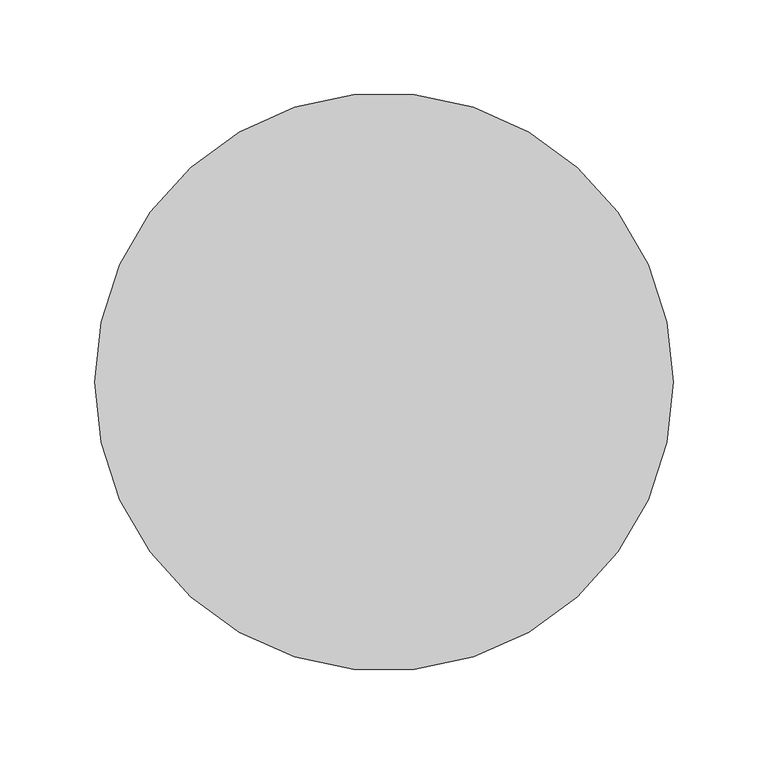
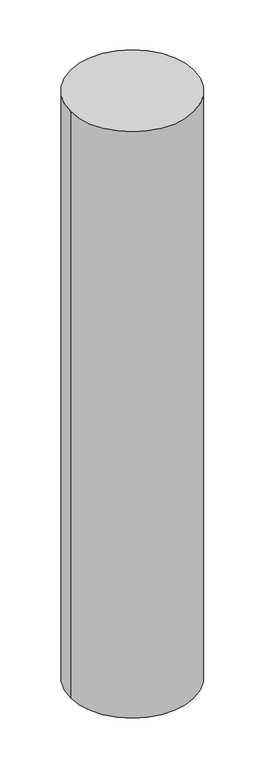
"""IFC4 building model written with IfcOpenShell, lengths in millimetres: proxy geometry."""

import ifcopenshell
import ifcopenshell.guid

model = None  # the IFC model being written
_history = None  # IfcOwnerHistory: only IFC2X3 demands one
_inside = {}  # id of a spatial element -> (the spatial element, [elements in it])
_under = {}  # id of a project, library or spatial element -> (it, [spatial elements below it])
_declared = {}  # id of a project -> (the project, [libraries it declares])
_typed = {}  # id of a type object -> (the type object, [elements of that type])
_made_of = {}  # id of a material, layer set ... -> (it, [elements and type objects made of it])


def new_model(schema):
    """Start an empty IFC model of exactly this schema.

    Asked for "IFC4X3", IfcOpenShell would pick the latest addendum, in which some entities
    have other attributes; the version numbers below select the first issue.
    IFC2X3 requires an IfcOwnerHistory on every rooted entity: one is made here for all.
    """
    global model, _history
    if schema == "IFC4X3":
        model = ifcopenshell.file(schema_version=(4, 3, 0, 0))
    else:
        model = ifcopenshell.file(schema=schema)
    _inside.clear()
    _under.clear()
    _declared.clear()
    _typed.clear()
    _made_of.clear()
    _history = None
    if model.schema == "IFC2X3":
        org = make("IfcOrganization", Name="unknown")
        user = make(
            "IfcPersonAndOrganization",
            ThePerson=make("IfcPerson", FamilyName="unknown"),
            TheOrganization=org,
        )
        app = make(
            "IfcApplication",
            ApplicationDeveloper=org,
            Version="unknown",
            ApplicationFullName="unknown",
            ApplicationIdentifier="unknown",
        )
        _history = make(
            "IfcOwnerHistory",
            OwningUser=user,
            OwningApplication=app,
            ChangeAction="ADDED",
            CreationDate=0,
        )
    return model


def make(cls, **values):
    """One entity of the class cls with the attributes given. An attribute that is None is left unset."""
    return model.create_entity(
        cls, **{name: value for name, value in values.items() if value is not None}
    )


def rooted(cls, **values):
    """An entity with a GlobalId (a new one), such as an element, a storey or a relation."""
    return make(cls, GlobalId=ifcopenshell.guid.new(), OwnerHistory=_history, **values)


def si_unit(unit_type, name, prefix=None):
    """IfcSIUnit, for example si_unit("LENGTHUNIT", "METRE", prefix="MILLI")."""
    return make("IfcSIUnit", UnitType=unit_type, Prefix=prefix, Name=name)


def assignment(units):
    """IfcUnitAssignment: the units of a project."""
    return None if units is None else make("IfcUnitAssignment", Units=units)


def point(xyz):
    """IfcCartesianPoint."""
    return None if xyz is None else make("IfcCartesianPoint", Coordinates=xyz)


def direction(xyz):
    """IfcDirection."""
    return None if xyz is None else make("IfcDirection", DirectionRatios=xyz)


def frame(location, z_axis=None, x_axis=None):
    """IfcAxis2Placement3D, a coordinate frame: its origin and axes. An axis left out is left unset."""
    return make(
        "IfcAxis2Placement3D",
        Location=point(location),
        Axis=direction(z_axis),
        RefDirection=direction(x_axis),
    )


def frame_2d(location, x_axis=None):
    """IfcAxis2Placement2D, a coordinate frame in the plane: its origin and x axis."""
    return make(
        "IfcAxis2Placement2D", Location=point(location), RefDirection=direction(x_axis)
    )


def origin():
    """The frame at (0, 0, 0) with its axes left unset."""
    return frame((0.0, 0.0, 0.0))


def place(relative_to, where):
    """IfcLocalPlacement: puts the frame where relative to a parent placement (None: the world)."""
    return make(
        "IfcLocalPlacement", PlacementRelTo=relative_to, RelativePlacement=where
    )


def context(
    kind, dimensions, precision=None, world=None, true_north=None, identifier=None
):
    """IfcGeometricRepresentationContext, for example the 3D "Model" context."""
    return make(
        "IfcGeometricRepresentationContext",
        ContextIdentifier=identifier,
        ContextType=kind,
        CoordinateSpaceDimension=dimensions,
        Precision=precision,
        WorldCoordinateSystem=world,
        TrueNorth=true_north,
    )


def project(units=None, contexts=None):
    """IfcProject with its units and contexts."""
    return rooted(
        "IfcProject",
        Name="project",
        RepresentationContexts=contexts,
        UnitsInContext=assignment(units),
    )


def spatial(cls, under=None, at=None, **own):
    """A site, building, storey or space (cls), placed at a placement, below another one or the project."""
    s = rooted(cls, ObjectPlacement=at, **own)
    if under is not None:
        _under.setdefault(under.id(), (under, []))[1].append(s)
    return s


def circle_curve(where, radius):
    """IfcCircle in the frame where."""
    return make("IfcCircle", Position=where, Radius=radius)


def trimmed(basis, trim1, trim2, sense, master):
    """IfcTrimmedCurve: the piece of a basis curve between two trims."""
    return make(
        "IfcTrimmedCurve",
        BasisCurve=basis,
        Trim1=trim1,
        Trim2=trim2,
        SenseAgreement=sense,
        MasterRepresentation=master,
    )


def segment(curve, same_sense, transition):
    """IfcCompositeCurveSegment."""
    return make(
        "IfcCompositeCurveSegment",
        Transition=transition,
        SameSense=same_sense,
        ParentCurve=curve,
    )


def composite_curve(segments, self_intersect=None):
    """IfcCompositeCurve: segments joined end to end."""
    return make("IfcCompositeCurve", Segments=segments, SelfIntersect=self_intersect)


def outline(outer, holes=None, kind="AREA"):
    """IfcArbitraryClosedProfileDef: a profile drawn as a closed curve; with holes, ...WithVoids."""
    if holes is None:
        return make("IfcArbitraryClosedProfileDef", ProfileType=kind, OuterCurve=outer)
    return make(
        "IfcArbitraryProfileDefWithVoids",
        ProfileType=kind,
        OuterCurve=outer,
        InnerCurves=holes,
    )


def extrude(swept, where, along, depth):
    """IfcExtrudedAreaSolid: the profile swept, set in the frame where, extruded along a direction by depth."""
    return make(
        "IfcExtrudedAreaSolid",
        SweptArea=swept,
        Position=where,
        ExtrudedDirection=direction(along),
        Depth=depth,
    )


def shape(context_of_items, identifier, shape_type, items):
    """IfcShapeRepresentation: the items that make up one representation, for example the "Body"."""
    return make(
        "IfcShapeRepresentation",
        ContextOfItems=context_of_items,
        RepresentationIdentifier=identifier,
        RepresentationType=shape_type,
        Items=items,
    )


def source(mapping_origin, context_of_items, identifier, shape_type, items):
    """IfcRepresentationMap: a shape defined once, which mapped items show again and again."""
    return make(
        "IfcRepresentationMap",
        MappingOrigin=mapping_origin,
        MappedRepresentation=shape(context_of_items, identifier, shape_type, items),
    )


def transform(
    local_origin,
    x_axis=None,
    y_axis=None,
    z_axis=None,
    scale=None,
    scale2=None,
    scale3=None,
    uniform=True,
):
    """IfcCartesianTransformationOperator3D, or its non-uniform kind. x_axis, y_axis, z_axis: its Axis1, 2, 3."""
    if uniform:
        return make(
            "IfcCartesianTransformationOperator3D",
            Axis1=direction(x_axis),
            Axis2=direction(y_axis),
            LocalOrigin=point(local_origin),
            Scale=scale,
            Axis3=direction(z_axis),
        )
    return make(
        "IfcCartesianTransformationOperator3DnonUniform",
        Axis1=direction(x_axis),
        Axis2=direction(y_axis),
        LocalOrigin=point(local_origin),
        Scale=scale,
        Axis3=direction(z_axis),
        Scale2=scale2,
        Scale3=scale3,
    )


def mapped(mapping_source, mapping_target):
    """IfcMappedItem: shows the shape of a source again, moved by a transform."""
    return make(
        "IfcMappedItem", MappingSource=mapping_source, MappingTarget=mapping_target
    )


def made_of(thing, what):
    """Note that an element or type object is made of a material, layer set ...; save() writes the relation."""
    if what is not None:
        _made_of.setdefault(what.id(), (what, []))[1].append(thing)
    return thing


def element(
    cls,
    number,
    at=None,
    inside=None,
    cuts=None,
    type_object=None,
    material=None,
    context=None,
    identifier="Body",
    shape_type=None,
    held_by="IfcProductDefinitionShape",
    body=None,
    shapes=None,
    **own,
):
    """One element of the class cls, such as IfcWall. Its Tag is "e" and its number.

    at: its placement. inside: the storey or other place that contains it. cuts: it is an
    opening in that element (IfcRelVoidsElement). A single representation is given by context,
    identifier, shape_type and body (its items); several are given by shapes. held_by: the class
    of the entity that holds the representations. save() writes the other relations.
    """
    e = rooted(cls, Tag="e%d" % number, ObjectPlacement=at, **own)
    if body is not None:
        shapes = [shape(context, identifier, shape_type, body)]
    if shapes is not None:
        e.Representation = make(held_by, Representations=shapes)
    if inside is not None:
        _inside.setdefault(inside.id(), (inside, []))[1].append(e)
    if cuts is not None:
        rooted(
            "IfcRelVoidsElement", RelatingBuildingElement=cuts, RelatedOpeningElement=e
        )
    if type_object is not None:
        _typed.setdefault(type_object.id(), (type_object, []))[1].append(e)
    return made_of(e, material)


def aggregate(whole, parts):
    """IfcRelAggregates: a whole, such as a stair, and the parts it consists of."""
    return rooted("IfcRelAggregates", RelatingObject=whole, RelatedObjects=parts)


def save(model, path):
    """Write the relations noted so far, then the file.

    IfcRelAggregates (storeys below a building ...), IfcRelContainedInSpatialStructure (elements
    in a storey), IfcRelDefinesByType, IfcRelAssociatesMaterial and IfcRelDeclares: one each for
    every whole, place, type object, material and project.
    """
    for whole, parts in _under.values():
        aggregate(whole, parts)
    for where, things in _inside.values():
        rooted(
            "IfcRelContainedInSpatialStructure",
            RelatedElements=things,
            RelatingStructure=where,
        )
    for kind, things in _typed.values():
        rooted("IfcRelDefinesByType", RelatedObjects=things, RelatingType=kind)
    for what, things in _made_of.values():
        rooted("IfcRelAssociatesMaterial", RelatedObjects=things, RelatingMaterial=what)
    for by, libraries in _declared.values():
        rooted("IfcRelDeclares", RelatingContext=by, RelatedDefinitions=libraries)
    model.write(path)


def generic_models_e1c0c775(model_context):
    return source(origin(), model_context, "Body", "SweptSolid", [
        extrude(outline(composite_curve([segment(trimmed(circle_curve(frame_2d((590220.6835267, -534045.8663841)), 152.4), [point((590068.2835267, -534045.8663841))], [point((590373.0835267, -534045.8663841))], False, "CARTESIAN"), True, "CONTINUOUS"), segment(trimmed(circle_curve(frame_2d((590220.6835267, -534045.8663841)), 152.4), [point((590373.0835267, -534045.8663841))], [point((590068.2835267, -534045.8663841))], False, "CARTESIAN"), True, "CONTINUOUS")], self_intersect=False)), frame((0.0, 0.0, -1676.4), z_axis=(0.0, 0.0, 1.0), x_axis=(1.0, 0.0, 0.0)), (0.0, 0.0, 1.0), 1524.0),
    ])


if __name__ == "__main__":
    model = new_model("IFC4")
    model_context = context("Model", 3, world=origin())
    ifc_project = project(units=[si_unit("LENGTHUNIT", "METRE", prefix="MILLI")], contexts=[model_context])
    site = spatial("IfcSite", under=ifc_project)
    building = spatial("IfcBuilding", under=site)
    placement = place(None, origin())
    generic_models_shape = generic_models_e1c0c775(model_context)
    element("IfcBuildingElementProxy", 1, Name="Sonotube Pier 2B1 : 12\" Sonotube Pier", ObjectType="Sonotube Pier 2B1 : 12\" Sonotube Pier", at=placement, inside=building, context=model_context, shape_type="MappedRepresentation", body=[
        mapped(generic_models_shape, transform((0.0, 0.0, 0.0), x_axis=(1.0, 0.0, 0.0), y_axis=(0.0, 1.0, 0.0), z_axis=(0.0, 0.0, 1.0))),
    ])
    save(model, "model.ifc")

# Revit data of these elements
# Element 1 (IfcBuildingElementProxy, "Sonotube Pier 2B1 : 12\" Sonotube Pier")
#   Materials on its faces: "12\" CONC SONOTUBE MIN. 60\" BELOW GRADE"
# Materials
#   "12\" CONC SONOTUBE MIN. 60\" BELOW GRADE": class "Generic", colour RGB 145 145 143, transparency 0, Cost = 0
